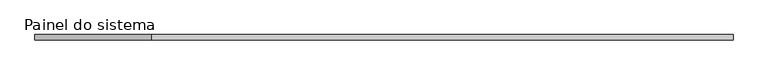
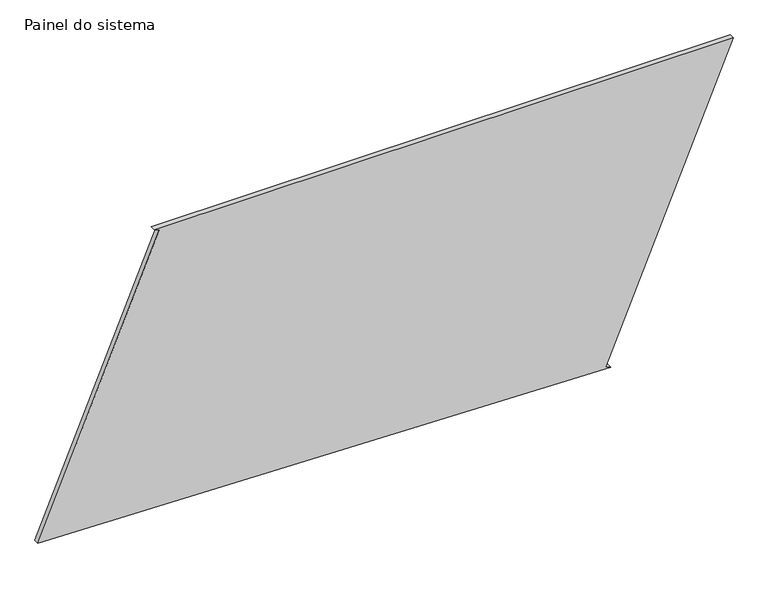
"""IFC4 building model written with IfcOpenShell, lengths in millimetres: plate geometry, Painel do sistema : Envidraçado."""

from ifc_helpers import new_model, si_unit, frame, origin, place, context, project, spatial, polyline, outline, extrude, source, transform, mapped, element, save


def painel_do_sistema_73bbb20a(model_context):
    return source(origin(), model_context, "Body", "SweptSolid", [
        extrude(outline(polyline([(0.0, 1074.9379067), (9.6723918, 1051.8848194), (1457.5378634, 1659.3662324), (1457.5378634, -1103.4187445), (1447.8654716, -1080.3656571), (67.8809602, -1659.3662324), (0.0, 1074.9379067)])), frame((0.0, 24.5, 0.0), z_axis=(0.0, 1.0, 0.0), x_axis=(0.0, 0.0, 1.0)), (0.0, 0.0, 1.0), 25.0),
    ])


if __name__ == "__main__":
    model = new_model("IFC4")
    model_context = context("Model", 3, world=origin())
    ifc_project = project(units=[si_unit("LENGTHUNIT", "METRE", prefix="MILLI")], contexts=[model_context])
    site = spatial("IfcSite", under=ifc_project)
    building = spatial("IfcBuilding", under=site)
    placement = place(None, origin())
    painel_do_sistema_shape = painel_do_sistema_73bbb20a(model_context)
    element("IfcPlate", 1, ObjectType="Painel do sistema : Envidraçado", at=placement, inside=building, context=model_context, shape_type="MappedRepresentation", body=[
        mapped(painel_do_sistema_shape, transform((0.0, 0.0, 0.0), x_axis=(1.0, 0.0, 0.0), y_axis=(0.0, 1.0, 0.0), z_axis=(0.0, 0.0, 1.0))),
    ])
    save(model, "model.ifc")

# Revit data of these elements
# Type "Painel do sistema : Envidraçado"
#   Construction Type Id = "GSP4R"
#   Analytic Construction = "Vidraça única Pilkington 1/8 pol"
#   Visual Light Transmittance = 0.9
#   Solar Heat Gain Coefficient = 0.86
#   Heat Transfer Coefficient (U) = 6.7069 W/(m²·K)
# Element 1 (IfcPlate, "Painel do sistema : Envidraçado")
#   Materials on its faces: "Vidro"
# Materials
#   "Vidro": class "Vidro", colour RGB 0 128 192, transparency 0.9, Description = "Vidro de sílica", Cost = 0
